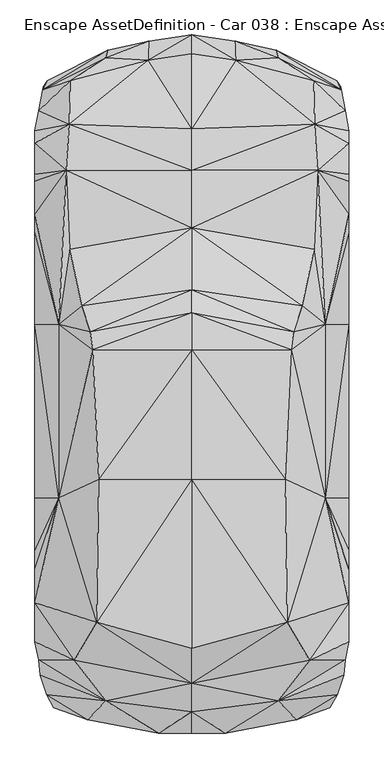
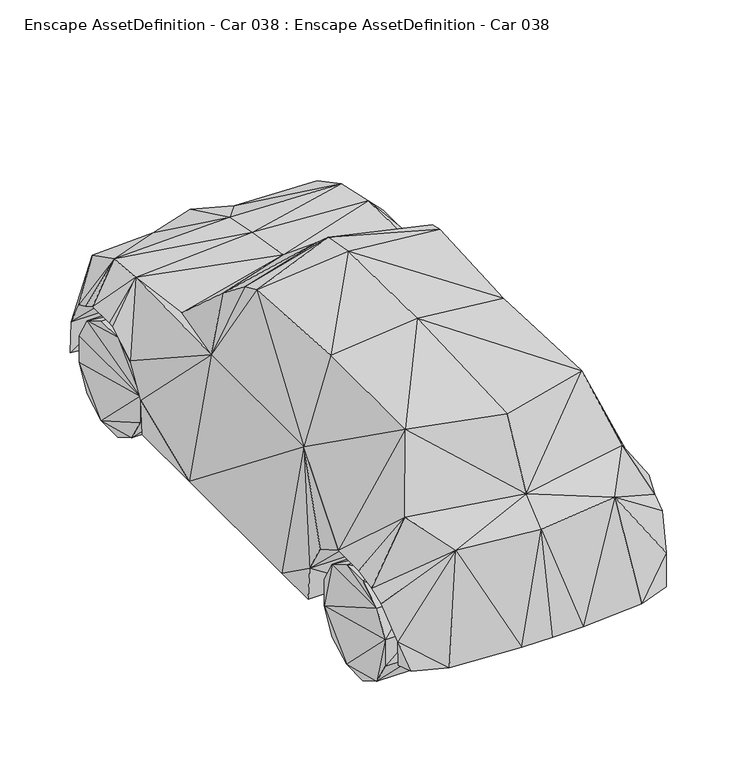
"""IFC4 building model written with IfcOpenShell, lengths in millimetres: geographic element geometry, Enscape AssetDefinition - Car 038 : Enscape AssetDefinition - Car 038."""

from ifc_helpers import new_model, si_unit, origin, place, context, project, spatial, faceted_brep, source, transform, mapped, element, save


def enscape_assetdefinition_car_038_enscape_assetdefinition_car_4a882751(model_context):
    return source(origin(), model_context, "Body", "Brep", [
        faceted_brep([(0.0, 1759.724021, 706.3940167), (0.0, 1362.8569841, 899.2630243), (232.9380065, 1725.1859903, 667.9729819), (0.0, 1141.2400007, 942.5449967), (652.5350213, 1384.9010468, 861.7839813), (-232.9380065, 1725.1859903, 667.9729819), (-652.5350213, 1384.9010468, 861.7839813), (0.0, 1860.4949713, 235.0659966), (-458.2389891, 1740.0100231, 589.1759992), (-647.6830244, 1615.6229973, 740.5700088), (-229.0029973, 1826.7560005, 228.2480001), (0.0, 1119.0090179, 228.7070006), (229.0029973, 1826.7560005, 228.2480001), (-448.7609863, 1779.2329788, 218.6439931), (-536.5399718, 1538.869977, 228.7070006), (-793.9119935, 1570.3920126, 415.2230024), (-813.9169812, 1457.7909708, 593.840003), (-536.5399718, 1570.3920126, 415.2230024), (-536.5409851, 1457.7909708, 593.840003), (-769.7229981, 1616.3719893, 218.6439931), (-790.6240225, 1583.7619305, 218.6439931), (-536.5399718, 1119.0090179, 228.7070006), (-536.5409851, 1283.5940123, 696.9649792), (-834.9990249, 1351.8069983, 656.5830112), (-834.9990249, 1283.5940123, 696.9649792), (-536.5409851, 1082.4500322, 696.9649792), (-834.9990249, 1119.0079451, 696.9649792), (-668.4240103, 1142.0849562, 901.4139771), (0.0, 834.1569901, 991.756022), (668.4240103, 1142.0849562, 901.4139771), (834.9990249, 1351.8069983, 656.5830112), (813.9169812, 1457.7909708, 593.840003), (647.6830244, 1615.6229973, 740.5700088), (834.9990249, 1283.5940123, 696.9649792), (793.9119935, 1570.3920126, 415.2230024), (536.5409851, 1457.7909708, 593.840003), (536.5409851, 1283.5940123, 696.9649792), (834.9990249, 1119.0079451, 696.9649792), (536.5409851, 1082.4500322, 696.9649792), (536.5399718, 1119.0090179, 228.7070006), (536.5399718, 1570.3920126, 415.2230024), (536.5399718, 1538.869977, 228.7070006), (790.6240225, 1583.7619305, 218.6439931), (448.7609863, 1779.2329788, 218.6439931), (769.7229981, 1616.3719893, 218.6439931), (458.2389891, 1740.0100231, 589.1759992), (0.0, 791.1509871, 215.9609944), (0.0, 322.3829865, 215.9609944), (-536.5399718, 791.1509871, 215.9609944), (536.5399718, 791.1509871, 215.9609944), (-536.5399718, 908.2540274, 593.840003), (-536.5399718, 807.6810241, 415.2219892), (-834.9980116, 807.6819777, 415.2230024), (-834.9980116, 908.2540274, 593.840003), (-834.9990249, 1082.4500322, 696.9649792), (-708.1069946, 322.3829865, 941.3419962), (-649.3980289, 720.0260162, 935.4360104), (-585.9040022, 420.4289913, 1213.778019), (649.3980289, 720.0260162, 935.4360104), (585.9040022, 420.4289913, 1213.778019), (0.0, 504.3359995, 1264.4159794), (-540.4459834, 281.7099988, 1321.7070103), (540.4459834, 281.7099988, 1321.7070103), (0.0, 383.4249973, 1372.344017), (708.1069946, 322.3829865, 941.3419962), (834.9990249, 1082.4500322, 696.9649792), (834.9980116, 908.2540274, 593.840003), (834.9980116, 807.6819777, 415.2230024), (536.5399718, 908.2540274, 593.840003), (536.5399718, 807.6810241, 415.2219892), (834.9990249, 791.1509871, 215.9609944), (834.9990249, 322.3829865, 215.9609944), (708.1069946, -600.063026, 941.3419962), (834.9990249, -600.063026, 215.9589976), (0.0, -600.063026, 215.9589976), (-834.9990249, 322.3829865, 215.9609944), (-834.9990249, 791.1509871, 215.9609944), (-708.1069946, -600.063026, 941.3419962), (-834.9990249, -600.063026, 215.9589976), (-526.7630219, 185.6089979, 1356.5779924), (0.0, 185.6089979, 1407.2149992), (-495.2780008, -501.4879704, 1364.1840219), (526.7630219, 185.6089979, 1356.5779924), (0.0, -501.4879704, 1414.8219824), (495.2780008, -501.4879704, 1364.1840219), (-506.8010092, -1262.9430294, 1380.8979988), (506.8010092, -1262.9430294, 1380.8979988), (0.0, -1399.5690346, 1380.8979988), (834.9990249, -1160.0530148, 696.9649792), (834.9990249, -981.4360142, 593.840003), (834.9990249, -878.3109784, 415.2219892), (536.5399718, -981.4350009, 593.8389897), (536.5399718, -1160.0530148, 696.9640255), (834.9990249, -861.3610268, 215.9589976), (536.5399718, -861.3610268, 215.9589976), (536.5399718, -878.3100247, 415.2219892), (536.5399718, -1461.8799686, 228.7060022), (0.0, -861.3610268, 215.9589976), (0.0, -1461.8799686, 228.7060022), (536.5399718, -1366.3020134, 696.9640255), (536.5399718, -1544.9199677, 593.840003), (834.9990249, -1366.3029671, 696.9649792), (813.9460087, -1461.8799686, 641.782999), (625.5189776, -1464.7020102, 1007.215023), (458.3640099, -1679.9800396, 880.6610107), (807.3629737, -1544.9199677, 593.840003), (0.0, -1587.3470306, 1007.215023), (-625.5189776, -1464.7020102, 1007.215023), (-458.3640099, -1679.9800396, 880.6610107), (0.0, -1737.0889187, 880.6610107), (-834.9990249, -1160.0530148, 696.9649792), (-834.9990249, -1366.3029671, 696.9649792), (-813.9460087, -1461.8799686, 641.782999), (-536.5399718, -1160.0530148, 696.9640255), (-536.5399718, -1366.3020134, 696.9640255), (-834.9990249, -981.4360142, 593.840003), (-834.9990249, -878.3109784, 415.2219892), (-536.5399718, -981.4350009, 593.8389897), (-536.5399718, -1461.8799686, 228.7060022), (-536.5399718, -878.3100247, 415.2219892), (-834.9990249, -861.3610268, 215.9589976), (-536.5399718, -861.3610268, 215.9589976), (0.0, -1851.6800404, 294.9950099), (177.2499979, -1851.6800404, 294.9950099), (-177.2499979, -1851.6800404, 294.9950099), (-554.7940135, -1781.0980082, 259.7180009), (-536.5399718, -1643.4259415, 265.3720081), (554.7940135, -1781.0980082, 259.7180009), (773.0429769, -1648.0439901, 415.2219892), (536.5399718, -1643.4259415, 265.3720081), (733.8359952, -1716.2730694, 263.7070119), (536.5399718, -1648.0439901, 415.2219892), (767.4019933, -1643.4259415, 265.3720081), (-807.3629737, -1544.9199677, 593.840003), (-773.0429769, -1648.0439901, 415.2219892), (-536.5399718, -1544.9199677, 593.840003), (-536.5399718, -1648.0439901, 415.2219892), (-767.4019933, -1643.4259415, 265.3720081), (-733.8359952, -1716.2730694, 263.7070119)], [[[0, 1, 2]], [[1, 3, 4]], [[0, 5, 1]], [[2, 1, 4]], [[1, 5, 6]], [[6, 3, 1]], [[0, 2, 7]], [[0, 7, 5]], [[8, 9, 5]], [[5, 9, 6]], [[10, 8, 5]], [[5, 7, 10]], [[11, 7, 12]], [[7, 2, 12]], [[11, 10, 7]], [[13, 8, 10]], [[14, 13, 10]], [[11, 14, 10]], [[8, 15, 9]], [[13, 15, 8]], [[16, 9, 15]], [[9, 16, 6]], [[17, 18, 15]], [[19, 15, 13]], [[15, 19, 20]], [[20, 17, 15]], [[15, 18, 16]], [[14, 19, 13]], [[19, 14, 20]], [[20, 14, 17]], [[21, 17, 14]], [[14, 11, 21]], [[21, 18, 17]], [[22, 23, 18]], [[21, 22, 18]], [[18, 23, 16]], [[6, 16, 23]], [[23, 22, 24]], [[24, 6, 23]], [[25, 26, 22]], [[21, 25, 22]], [[22, 26, 24]], [[26, 27, 24]], [[24, 27, 6]], [[27, 3, 6]], [[3, 28, 29]], [[3, 27, 28]], [[4, 3, 29]], [[30, 31, 4]], [[4, 32, 2]], [[30, 4, 33]], [[4, 29, 33]], [[4, 31, 32]], [[34, 32, 31]], [[31, 30, 35]], [[31, 35, 34]], [[33, 36, 30]], [[35, 30, 36]], [[33, 37, 36]], [[33, 29, 37]], [[36, 38, 39]], [[35, 36, 39]], [[36, 37, 38]], [[40, 35, 39]], [[34, 35, 40]], [[41, 40, 39]], [[34, 40, 42]], [[40, 41, 42]], [[11, 41, 39]], [[41, 12, 43]], [[41, 11, 12]], [[41, 43, 44]], [[41, 44, 42]], [[42, 44, 34]], [[44, 43, 34]], [[43, 12, 45]], [[34, 43, 45]], [[45, 12, 2]], [[2, 32, 45]], [[32, 34, 45]], [[11, 39, 46]], [[11, 46, 21]], [[46, 47, 48]], [[49, 47, 46]], [[46, 39, 49]], [[21, 46, 48]], [[21, 50, 25]], [[51, 21, 48]], [[21, 51, 50]], [[51, 52, 50]], [[50, 53, 25]], [[50, 52, 53]], [[26, 25, 54]], [[25, 53, 54]], [[52, 55, 53]], [[53, 27, 54]], [[53, 55, 27]], [[54, 27, 26]], [[55, 56, 27]], [[28, 27, 56]], [[55, 57, 56]], [[57, 28, 56]], [[58, 28, 59]], [[60, 28, 57]], [[59, 28, 60]], [[29, 28, 58]], [[55, 61, 57]], [[61, 60, 57]], [[59, 60, 62]], [[63, 60, 61]], [[62, 60, 63]], [[59, 62, 64]], [[58, 59, 64]], [[29, 58, 64]], [[37, 29, 65]], [[65, 29, 66]], [[29, 64, 66]], [[65, 66, 38]], [[65, 38, 37]], [[66, 64, 67]], [[67, 68, 66]], [[38, 66, 68]], [[38, 68, 39]], [[69, 68, 67]], [[68, 69, 39]], [[70, 49, 67]], [[64, 71, 67]], [[70, 67, 71]], [[67, 49, 69]], [[49, 39, 69]], [[70, 71, 49]], [[71, 47, 49]], [[64, 72, 71]], [[73, 74, 71]], [[71, 72, 73]], [[71, 74, 47]], [[48, 47, 75]], [[74, 75, 47]], [[76, 52, 48]], [[48, 75, 76]], [[48, 52, 51]], [[52, 75, 55]], [[75, 52, 76]], [[55, 75, 77]], [[78, 75, 74]], [[77, 75, 78]], [[55, 79, 61]], [[77, 79, 55]], [[80, 63, 79]], [[81, 79, 77]], [[79, 63, 61]], [[81, 80, 79]], [[80, 82, 63]], [[63, 82, 62]], [[83, 84, 80]], [[83, 80, 81]], [[80, 84, 82]], [[81, 77, 85]], [[85, 83, 81]], [[84, 83, 86]], [[87, 83, 85]], [[86, 83, 87]], [[86, 72, 84]], [[84, 72, 82]], [[62, 82, 64]], [[82, 72, 64]], [[88, 89, 72]], [[72, 86, 88]], [[73, 72, 90]], [[90, 72, 89]], [[89, 91, 90]], [[88, 92, 89]], [[89, 92, 91]], [[93, 90, 94]], [[93, 73, 90]], [[90, 91, 95]], [[94, 90, 95]], [[93, 94, 73]], [[73, 94, 74]], [[94, 95, 96]], [[97, 94, 98]], [[98, 94, 96]], [[74, 94, 97]], [[95, 91, 96]], [[91, 92, 96]], [[92, 99, 96]], [[88, 99, 92]], [[99, 100, 96]], [[101, 99, 88]], [[101, 102, 99]], [[99, 102, 100]], [[101, 88, 103]], [[88, 86, 103]], [[102, 101, 103]], [[104, 105, 102]], [[105, 100, 102]], [[104, 102, 103]], [[103, 106, 104]], [[86, 106, 103]], [[87, 106, 86]], [[87, 85, 106]], [[107, 108, 106]], [[104, 106, 109]], [[106, 85, 107]], [[106, 108, 109]], [[77, 110, 85]], [[85, 110, 107]], [[107, 111, 112]], [[107, 110, 111]], [[112, 108, 107]], [[113, 114, 110]], [[77, 115, 110]], [[110, 114, 111]], [[115, 113, 110]], [[116, 77, 78]], [[115, 77, 116]], [[117, 113, 115]], [[116, 117, 115]], [[118, 114, 113]], [[118, 113, 117]], [[119, 117, 116]], [[118, 117, 119]], [[120, 121, 116]], [[116, 78, 120]], [[116, 121, 119]], [[78, 121, 120]], [[74, 121, 78]], [[118, 119, 121]], [[97, 98, 121]], [[97, 121, 74]], [[121, 98, 118]], [[122, 98, 123]], [[122, 124, 98]], [[123, 98, 96]], [[98, 124, 118]], [[123, 109, 122]], [[124, 122, 109]], [[124, 108, 125]], [[126, 124, 125]], [[124, 126, 118]], [[124, 109, 108]], [[123, 104, 109]], [[104, 123, 127]], [[128, 104, 127]], [[104, 128, 105]], [[127, 129, 130]], [[127, 123, 129]], [[128, 127, 130]], [[129, 96, 131]], [[96, 129, 123]], [[131, 132, 129]], [[130, 129, 132]], [[130, 132, 128]], [[128, 132, 131]], [[105, 128, 100]], [[100, 128, 131]], [[100, 131, 96]], [[133, 108, 112]], [[108, 133, 134]], [[125, 108, 134]], [[112, 135, 133]], [[135, 112, 114]], [[114, 112, 111]], [[135, 134, 133]], [[118, 135, 114]], [[118, 136, 135]], [[136, 134, 135]], [[136, 118, 126]], [[126, 137, 136]], [[136, 137, 134]], [[137, 126, 138]], [[138, 126, 125]], [[125, 134, 138]], [[134, 137, 138]]]),
        faceted_brep([(799.5659709, -1183.9879751, 3.5600001), (799.5659709, -962.0429873, 225.503996), (799.5659709, -1568.4039593, 387.9779875), (799.5659709, -1043.2800055, 84.7970024), (612.7390265, -1043.2800055, 84.7970024), (799.5659709, -962.0440006, 387.9779875), (612.7390265, -962.0429873, 387.9770041), (799.5659709, -1487.1670008, 528.68402), (612.7390265, -962.0429873, 225.503996), (612.7390265, -1183.9879751, 3.5600001), (612.7390265, -1568.4039593, 387.9770041), (612.7390265, -1183.9870214, 609.9200249), (612.7390265, -1043.2809591, 528.68402), (612.7390265, -1487.1670008, 84.7970024), (612.7390265, -1346.4610577, 3.5600001), (612.7390265, -1568.4039593, 225.503996), (799.5659709, -1043.2809591, 528.68402), (799.5659709, -1183.9879751, 609.9209785), (799.5659709, -1346.4610577, 609.9209785), (612.7390265, -1346.4610577, 609.9200249), (612.7390265, -1487.1670008, 528.68402), (799.5659709, -1568.4039593, 225.503996), (799.5659709, -1487.1670008, 84.7970024), (799.5659709, -1346.4610577, 3.5600001)], [[[0, 1, 2]], [[3, 4, 1]], [[5, 1, 6]], [[7, 1, 5]], [[1, 7, 2]], [[1, 0, 3]], [[1, 4, 8]], [[6, 1, 8]], [[9, 8, 4]], [[3, 9, 4]], [[0, 9, 3]], [[9, 10, 11]], [[9, 12, 6]], [[9, 6, 8]], [[13, 9, 14]], [[9, 13, 15]], [[9, 15, 10]], [[9, 11, 12]], [[0, 14, 9]], [[16, 5, 12]], [[12, 5, 6]], [[11, 16, 12]], [[17, 16, 11]], [[7, 5, 16]], [[7, 16, 17]], [[18, 17, 19]], [[7, 17, 18]], [[19, 17, 11]], [[7, 18, 20]], [[2, 7, 10]], [[10, 7, 20]], [[20, 18, 19]], [[19, 10, 20]], [[10, 19, 11]], [[2, 10, 21]], [[21, 10, 15]], [[22, 2, 21]], [[0, 2, 22]], [[21, 15, 22]], [[22, 15, 13]], [[22, 13, 23]], [[0, 22, 23]], [[23, 14, 0]], [[23, 13, 14]]]),
        faceted_brep([(799.5659709, 1258.6860657, 3.8600001), (799.5659709, 1480.6300402, 225.8030027), (799.5659709, 874.2700219, 388.2760108), (799.5659709, 1399.3929625, 85.0960016), (612.7390265, 1480.6300402, 225.8020043), (799.5659709, 1480.6300402, 388.2760108), (612.7390265, 1258.6860657, 3.8600001), (612.7390265, 1399.3929625, 85.0960016), (612.7399802, 1096.2120295, 610.220015), (612.7390265, 1480.6300402, 388.2760108), (799.5659709, 1399.3929625, 528.9829969), (612.7399802, 1399.3929625, 528.9829969), (612.7399802, 1258.6860657, 610.220015), (799.5659709, 1258.6860657, 610.220015), (799.5659709, 1096.2129831, 610.220015), (799.5659709, 955.5060267, 528.9819837), (612.7390265, 874.2700219, 388.2760108), (799.5659709, 874.2700219, 225.8020043), (612.7390265, 955.5060267, 528.9819837), (612.7390265, 874.2700219, 225.8020043), (799.5659709, 955.5060267, 85.0960016), (799.5659709, 1096.2120295, 3.859), (612.7390265, 1096.2120295, 3.859), (612.7390265, 955.5060267, 85.0960016)], [[[0, 1, 2]], [[1, 3, 4]], [[1, 4, 5]], [[2, 1, 5]], [[1, 0, 3]], [[0, 6, 3]], [[4, 3, 7]], [[3, 6, 7]], [[8, 9, 4]], [[6, 4, 7]], [[8, 4, 6]], [[5, 4, 9]], [[10, 5, 11]], [[2, 5, 10]], [[11, 5, 9]], [[8, 11, 9]], [[11, 8, 12]], [[12, 10, 11]], [[13, 10, 12]], [[14, 10, 13]], [[2, 10, 14]], [[13, 12, 14]], [[14, 12, 8]], [[14, 8, 15]], [[2, 14, 15]], [[2, 15, 16]], [[2, 16, 17]], [[0, 2, 17]], [[15, 8, 18]], [[16, 15, 18]], [[6, 16, 8]], [[6, 19, 16]], [[8, 16, 18]], [[17, 16, 19]], [[17, 19, 20]], [[0, 17, 20]], [[21, 22, 0]], [[0, 20, 21]], [[0, 22, 6]], [[23, 6, 22]], [[6, 23, 19]], [[20, 19, 23]], [[20, 23, 21]], [[21, 23, 22]]]),
        faceted_brep([(-799.5659709, -1568.3810711, 388.3619905), (-799.5659709, -1183.9640141, 3.945), (-799.5659709, -1487.1439934, 85.1820037), (-799.5659709, -1346.4379311, 3.945), (-612.7390265, -1346.4379311, 3.945), (-799.5659709, -1043.2569981, 85.1820037), (-612.7390265, -1183.9640141, 3.945), (-799.5659709, -962.01998, 225.8879989), (-612.7390265, -1487.1439934, 85.1820037), (-612.7390265, -1568.3810711, 388.361007), (-612.7390265, -1568.3810711, 225.8879989), (-612.7390265, -962.01998, 225.8879989), (-612.7390265, -1043.2569981, 85.1809978), (-612.7390265, -962.01998, 388.361007), (-612.7390265, -1183.9640141, 610.303998), (-799.5659709, -962.0209932, 388.3619905), (-612.7390265, -1043.2579517, 529.0679932), (-799.5659709, -1043.2579517, 529.0679932), (-799.5659709, -1183.9649677, 610.3050113), (-612.7390265, -1346.4379311, 610.303998), (-799.5659709, -1487.1439934, 529.0679932), (-799.5659709, -1346.4379311, 610.3050113), (-612.7390265, -1487.1439934, 529.0679932), (-799.5659709, -1568.3810711, 225.8879989)], [[[0, 1, 2]], [[3, 1, 4]], [[1, 5, 6]], [[1, 7, 5]], [[2, 1, 3]], [[0, 7, 1]], [[4, 1, 6]], [[8, 3, 4]], [[6, 8, 4]], [[2, 3, 8]], [[8, 9, 10]], [[6, 9, 8]], [[10, 2, 8]], [[6, 11, 9]], [[11, 6, 12]], [[6, 5, 12]], [[5, 7, 12]], [[12, 7, 11]], [[11, 7, 13]], [[14, 11, 13]], [[9, 11, 14]], [[13, 15, 16]], [[14, 13, 16]], [[13, 7, 15]], [[16, 17, 14]], [[14, 18, 19]], [[9, 14, 19]], [[14, 17, 18]], [[16, 15, 17]], [[7, 17, 15]], [[18, 17, 20]], [[20, 17, 7]], [[18, 20, 21]], [[19, 18, 21]], [[19, 21, 22]], [[9, 19, 22]], [[22, 21, 20]], [[20, 0, 22]], [[7, 0, 20]], [[22, 0, 9]], [[0, 23, 9]], [[9, 23, 10]], [[0, 2, 23]], [[23, 2, 10]]]),
        faceted_brep([(-799.5659709, 1399.3929625, 528.9829969), (-799.5659709, 874.2700219, 388.2760108), (-799.5659709, 1096.2129831, 610.220015), (-799.5659709, 874.2700219, 225.8020043), (-612.7390265, 874.2700219, 388.2760108), (-799.5659709, 1480.6300402, 388.2760108), (-799.5659709, 1480.6300402, 225.8030027), (-799.5659709, 1258.6860657, 3.8600001), (-799.5659709, 955.5060267, 528.9819837), (-799.5659709, 955.5060267, 85.0960016), (-612.7390265, 874.2700219, 225.8020043), (-799.5659709, 1096.2120295, 3.859), (-612.7390265, 955.5060267, 85.0960016), (-612.7390265, 1258.6860657, 3.8600001), (-612.7390265, 1096.2120295, 3.859), (-612.7390265, 1096.2120295, 610.220015), (-612.7390265, 1480.6300402, 225.8020043), (-612.7390265, 1399.3929625, 85.0960016), (-799.5659709, 1399.3929625, 85.0960016), (-612.7390265, 1480.6300402, 388.2760108), (-612.7390265, 1399.3929625, 528.9829969), (-612.7390265, 1258.6860657, 610.220015), (-799.5659709, 1258.6860657, 610.220015), (-612.7390265, 955.5060267, 528.9819837)], [[[0, 1, 2]], [[1, 3, 4]], [[1, 0, 5]], [[1, 5, 6]], [[7, 3, 1]], [[2, 1, 8]], [[1, 6, 7]], [[4, 8, 1]], [[3, 9, 10]], [[7, 9, 3]], [[4, 3, 10]], [[9, 11, 12]], [[9, 7, 11]], [[10, 9, 12]], [[13, 4, 10]], [[13, 10, 12]], [[13, 12, 14]], [[12, 11, 14]], [[11, 7, 14]], [[14, 7, 13]], [[15, 13, 16]], [[13, 7, 17]], [[16, 13, 17]], [[13, 15, 4]], [[17, 18, 16]], [[17, 7, 18]], [[7, 6, 18]], [[16, 18, 6]], [[6, 5, 16]], [[15, 16, 19]], [[16, 5, 19]], [[19, 5, 20]], [[20, 5, 0]], [[15, 19, 20]], [[20, 0, 21]], [[15, 20, 21]], [[0, 2, 22]], [[21, 0, 22]], [[22, 2, 21]], [[21, 2, 15]], [[2, 8, 15]], [[4, 15, 23]], [[15, 8, 23]], [[23, 8, 4]]]),
    ])


if __name__ == "__main__":
    model = new_model("IFC4")
    model_context = context("Model", 3, world=origin())
    ifc_project = project(units=[si_unit("LENGTHUNIT", "METRE", prefix="MILLI")], contexts=[model_context])
    site = spatial("IfcSite", under=ifc_project)
    building = spatial("IfcBuilding", under=site)
    placement = place(None, origin())
    enscape_assetdefinition_car_038_enscape_assetdefinition_car_shape = enscape_assetdefinition_car_038_enscape_assetdefinition_car_4a882751(model_context)
    element("IfcGeographicElement", 1, ObjectType="Enscape AssetDefinition - Car 038 : Enscape AssetDefinition - Car 038", at=placement, inside=building, context=model_context, shape_type="MappedRepresentation", body=[
        mapped(enscape_assetdefinition_car_038_enscape_assetdefinition_car_shape, transform((0.0, 0.0, 0.0), x_axis=(1.0, 0.0, 0.0), y_axis=(0.0, 1.0, 0.0), z_axis=(0.0, 0.0, 1.0))),
    ])
    save(model, "model.ifc")

# Revit data of these elements
# Type "Enscape AssetDefinition - Car 038 : Enscape AssetDefinition - Car 038"
#   EnscapeAssetSource = "REMOTE"
#   EnscapeAssetId = "57b9b5da-9f20-40da-9c13-bb8bf671bc5a"
#   Height = 1414.822 mm
#   EnscapeNativeAssetHeight = 1414.822 mm
#   Default Elevation = 0
